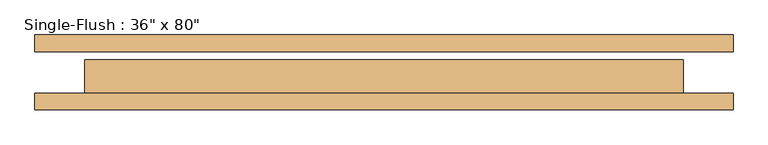
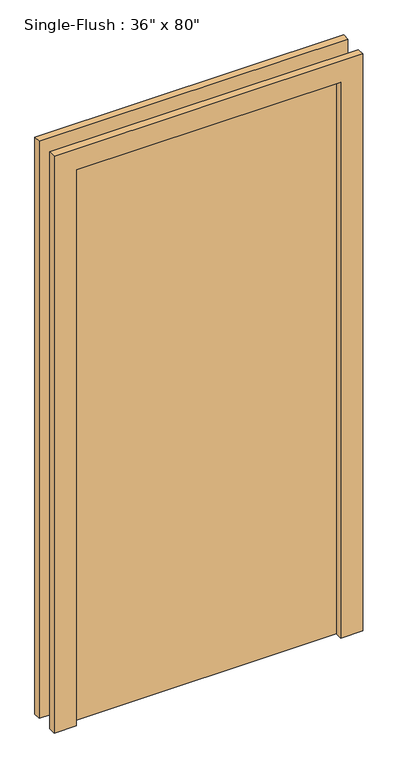
"""IFC4 building model written with IfcOpenShell, lengths in millimetres: door geometry."""

from ifc_helpers import new_model, si_unit, frame, origin, origin_with_axes, place, context, project, spatial, polyline, outline, extrude, source, transform, mapped, element, save


def door_9886d463(model_context):
    return source(origin(), model_context, "Body", "SweptSolid", [
        extrude(outline(polyline([(2108.2, -533.4), (0.0, -533.4), (0.0, -457.2), (2032.0, -457.2), (2032.0, 457.2), (0.0, 457.2), (0.0, 533.4), (2108.2, 533.4), (2108.2, -533.4)])), frame((0.0, -57.15, 0.0), z_axis=(0.0, 1.0, 0.0), x_axis=(0.0, 0.0, 1.0)), (0.0, 0.0, 1.0), 25.4),
        extrude(outline(polyline([(2108.2, 533.4), (2108.2, -533.4), (0.0, -533.4), (0.0, -457.2), (2032.0, -457.2), (2032.0, 457.2), (0.0, 457.2), (0.0, 533.4), (2108.2, 533.4)])), frame((0.0, 31.75, 0.0), z_axis=(0.0, 1.0, 0.0), x_axis=(0.0, 0.0, 1.0)), (0.0, 0.0, 1.0), 25.4),
        extrude(outline(polyline([(457.2, 19.05), (457.2, -31.75), (-457.2, -31.75), (-457.2, 19.05), (457.2, 19.05)])), origin_with_axes(), (0.0, 0.0, 1.0), 2032.0),
    ])


if __name__ == "__main__":
    model = new_model("IFC4")
    model_context = context("Model", 3, world=origin())
    ifc_project = project(units=[si_unit("LENGTHUNIT", "METRE", prefix="MILLI")], contexts=[model_context])
    site = spatial("IfcSite", under=ifc_project)
    building = spatial("IfcBuilding", under=site)
    placement = place(None, origin())
    door_shape = door_9886d463(model_context)
    element("IfcDoor", 1, ObjectType="Single-Flush : 36\" x 80\"", at=placement, inside=building, context=model_context, shape_type="MappedRepresentation", body=[
        mapped(door_shape, transform((0.0, 0.0, 0.0), x_axis=(1.0, 0.0, 0.0), y_axis=(0.0, 1.0, 0.0), z_axis=(0.0, 0.0, 1.0))),
    ])
    save(model, "model.ifc")

# Revit data of these elements
# Type "Single-Flush : 36\" x 80\""
#   Type Mark = "6"
#   Construction Type Id = "MDOOR"
#   Assembly Code = "C1020"
#   Analytic Construction = "Metal"
#   Thickness = 0' - 2"
#   Heat Transfer Coefficient (U) = 0.651978 BTU/(h·ft²·°F)
#   Height = 6' - 8"
#   Trim Projection Ext = 0' - 1"
#   Trim Projection Int = 0' - 1"
#   Trim Width = 0' - 3"
#   Width = 3' - 0"
#   Define Thermal Properties by = 1
#   Define Thermal Properties by = 1
#   Door Material = Door - Panel
#   Frame Material = Door - Frame
#   Visual Light Transmittance = 0
#   Solar Heat Gain Coefficient = 0
#   Function = (empty or 0)
#   Wall Closure = (empty or 0)
# Element 1 (IfcDoor, "Single-Flush : 36\" x 80\"")
#   Materials on its faces: "Door - Frame", "Door - Panel"
# Materials
#   "Door - Panel": class "Wood", colour RGB 210 159 95, transparency 0, Cost = 0
#   "Door - Frame": class "Miscellaneous", colour RGB 118 70 51, transparency 0, Cost = 0
